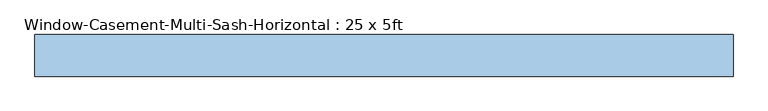
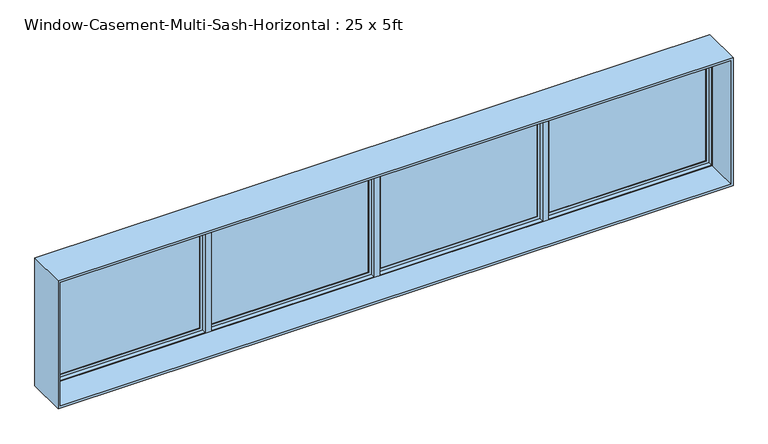
"""IFC4 building model written with IfcOpenShell, lengths in millimetres: window geometry, Window-Casement-Multi-Sash-Horizontal : 25 x 5ft."""

from ifc_helpers import new_model, si_unit, frame, origin, place, context, project, spatial, polyline, outline, extrude, faceted_brep, source, transform, mapped, element, save


def window_casement_multi_sash_horizontal_25_x_5ft_0e5d08e3(model_context):
    return source(origin(), model_context, "Body", "SolidModel", [
        extrude(outline(polyline([(2413.0, -1879.6), (939.8, -1879.6), (939.8, -25.4), (2413.0, -25.4), (2413.0, -1879.6)]), holes=[polyline([(2371.1296875, -67.2703125), (981.6703125, -67.2703125), (981.6703125, -1837.7296875), (2371.1296875, -1837.7296875), (2371.1296875, -67.2703125)])]), frame((0.0, 185.7375, 0.0), z_axis=(0.0, 1.0, 0.0), x_axis=(0.0, 0.0, 1.0)), (0.0, 0.0, 1.0), 31.75),
        extrude(outline(polyline([(2413.0, 25.4), (939.8, 25.4), (939.8, 1879.6), (2413.0, 1879.6), (2413.0, 25.4)]), holes=[polyline([(2371.1296875, 1837.7296875), (981.6703125, 1837.7296875), (981.6703125, 67.2703125), (2371.1296875, 67.2703125), (2371.1296875, 1837.7296875)])]), frame((0.0, 185.7375, 0.0), z_axis=(0.0, 1.0, 0.0), x_axis=(0.0, 0.0, 1.0)), (0.0, 0.0, 1.0), 31.75),
        faceted_brep([(-1930.4, 185.7375, 2413.0), (-3784.6, 185.7375, 2413.0), (-3784.6, 227.0125, 2413.0), (3784.6, 227.0125, 2413.0), (3784.6, 185.7375, 2413.0), (1930.4, 185.7375, 2413.0), (1930.4, 223.8375, 2413.0), (1879.6, 223.8375, 2413.0), (1879.6, 185.7375, 2413.0), (25.4, 185.7375, 2413.0), (25.4, 223.8375, 2413.0), (-25.4, 223.8375, 2413.0), (-25.4, 185.7375, 2413.0), (-1879.6, 185.7375, 2413.0), (-1879.6, 223.8375, 2413.0), (-1930.4, 223.8375, 2413.0), (-3774.4796875, 134.9375, 2402.8796875), (-3774.4796875, 185.7375, 2402.8796875), (-1940.5203125, 185.7375, 2402.8796875), (-1940.5203125, 134.9375, 2402.8796875), (3774.4796875, 185.7375, 2402.8796875), (3774.4796875, 134.9375, 2402.8796875), (1940.5203125, 134.9375, 2402.8796875), (1940.5203125, 185.7375, 2402.8796875), (-1869.4796875, 185.7375, 2402.8796875), (-35.5203125, 185.7375, 2402.8796875), (-35.5203125, 134.9375, 2402.8796875), (-1869.4796875, 134.9375, 2402.8796875), (35.5203125, 185.7375, 2402.8796875), (1869.4796875, 185.7375, 2402.8796875), (1869.4796875, 134.9375, 2402.8796875), (35.5203125, 134.9375, 2402.8796875), (-3784.6, -227.0125, 2413.0), (-3784.6, 134.9375, 2413.0), (3784.6, 134.9375, 2413.0), (3784.6, -227.0125, 2413.0), (-3810.0, 227.0125, 2438.4), (-3810.0, -227.0125, 2438.4), (3810.0, -227.0125, 2438.4), (3810.0, 227.0125, 2438.4), (3784.6, 227.0125, 939.8), (3784.6, 185.7375, 939.8), (3774.4796875, 185.7375, 949.9203125), (3774.4796875, 134.9375, 949.9203125), (3784.6, 134.9375, 939.8), (3784.6, -227.0125, 939.8), (3810.0, -227.0125, 914.4), (3810.0, 227.0125, 914.4), (1930.4, 185.7375, 939.8), (-3784.6, 227.0125, 939.8), (-3784.6, 185.7375, 939.8), (-1930.4, 185.7375, 939.8), (-1930.4, 223.8375, 939.8), (-1879.6, 223.8375, 939.8), (-1879.6, 185.7375, 939.8), (-25.4, 185.7375, 939.8), (-25.4, 223.8375, 939.8), (25.4, 223.8375, 939.8), (25.4, 185.7375, 939.8), (1879.6, 185.7375, 939.8), (1879.6, 223.8375, 939.8), (1930.4, 223.8375, 939.8), (1940.5203125, 185.7375, 949.9203125), (1940.5203125, 134.9375, 949.9203125), (-3774.4796875, 185.7375, 949.9203125), (-3774.4796875, 134.9375, 949.9203125), (-1940.5203125, 134.9375, 949.9203125), (-1940.5203125, 185.7375, 949.9203125), (-35.5203125, 185.7375, 949.9203125), (-1869.4796875, 185.7375, 949.9203125), (-1869.4796875, 134.9375, 949.9203125), (-35.5203125, 134.9375, 949.9203125), (1869.4796875, 185.7375, 949.9203125), (35.5203125, 185.7375, 949.9203125), (35.5203125, 134.9375, 949.9203125), (1869.4796875, 134.9375, 949.9203125), (-3784.6, 134.9375, 939.8), (-3784.6, -227.0125, 939.8), (-3810.0, -227.0125, 914.4), (-3810.0, 227.0125, 914.4)], [[[0, 1, 2, 3, 4, 5, 6, 7, 8, 9, 10, 11, 12, 13, 14, 15]], [[16, 17, 18, 19]], [[20, 21, 22, 23]], [[24, 25, 26, 27]], [[28, 29, 30, 31]], [[32, 33, 34, 35]], [[36, 37, 38, 39]], [[4, 3, 40, 41]], [[21, 20, 42, 43]], [[35, 34, 44, 45]], [[39, 38, 46, 47]], [[48, 41, 40, 49, 50, 51, 52, 53, 54, 55, 56, 57, 58, 59, 60, 61]], [[43, 42, 62, 63]], [[64, 65, 66, 67]], [[68, 69, 70, 71]], [[72, 73, 74, 75]], [[45, 44, 76, 77]], [[47, 46, 78, 79]], [[2, 1, 50, 49]], [[4, 41, 48, 5], [20, 23, 62, 42]], [[50, 1, 0, 51], [64, 67, 18, 17]], [[12, 55, 54, 13], [69, 68, 25, 24]], [[8, 59, 58, 9], [73, 72, 29, 28]], [[17, 16, 65, 64]], [[44, 34, 33, 76], [16, 19, 66, 65], [27, 26, 71, 70], [31, 30, 75, 74], [21, 43, 63, 22]], [[33, 32, 77, 76]], [[38, 37, 78, 46], [32, 35, 45, 77]], [[37, 36, 79, 78]], [[36, 39, 47, 79], [3, 2, 49, 40]], [[18, 67, 66, 19]], [[69, 24, 27, 70]], [[53, 14, 13, 54]], [[14, 53, 52, 15]], [[15, 52, 51, 0]], [[25, 68, 71, 26]], [[73, 28, 31, 74]], [[57, 10, 9, 58]], [[10, 57, 56, 11]], [[11, 56, 55, 12]], [[6, 61, 60, 7]], [[7, 60, 59, 8]], [[29, 72, 75, 30]], [[62, 23, 22, 63]], [[61, 6, 5, 48]]]),
        extrude(outline(polyline([(-67.2703125, 211.1375), (-67.2703125, 204.7875), (-1837.7296875, 204.7875), (-1837.7296875, 211.1375), (-67.2703125, 211.1375)])), frame((0.0, 0.0, 981.6703125), z_axis=(0.0, 0.0, 1.0), x_axis=(1.0, 0.0, 0.0)), (0.0, 0.0, 1.0), 1389.459375),
        extrude(outline(polyline([(-67.2703125, 198.4375), (-67.2703125, 192.0875), (-1837.7296875, 192.0875), (-1837.7296875, 198.4375), (-67.2703125, 198.4375)])), frame((0.0, 0.0, 981.6703125), z_axis=(0.0, 0.0, 1.0), x_axis=(1.0, 0.0, 0.0)), (0.0, 0.0, 1.0), 1389.459375),
        extrude(outline(polyline([(1837.7296875, 211.1375), (1837.7296875, 204.7875), (67.2703125, 204.7875), (67.2703125, 211.1375), (1837.7296875, 211.1375)])), frame((0.0, 0.0, 981.6703125), z_axis=(0.0, 0.0, 1.0), x_axis=(1.0, 0.0, 0.0)), (0.0, 0.0, 1.0), 1389.459375),
        extrude(outline(polyline([(1837.7296875, 198.4375), (1837.7296875, 192.0875), (67.2703125, 192.0875), (67.2703125, 198.4375), (1837.7296875, 198.4375)])), frame((0.0, 0.0, 981.6703125), z_axis=(0.0, 0.0, 1.0), x_axis=(1.0, 0.0, 0.0)), (0.0, 0.0, 1.0), 1389.459375),
        extrude(outline(polyline([(-1972.2703125, 211.1375), (-1972.2703125, 204.7875), (-3742.7296875, 204.7875), (-3742.7296875, 211.1375), (-1972.2703125, 211.1375)])), frame((0.0, 0.0, 981.6703125), z_axis=(0.0, 0.0, 1.0), x_axis=(1.0, 0.0, 0.0)), (0.0, 0.0, 1.0), 1389.459375),
        extrude(outline(polyline([(-1972.2703125, 198.4375), (-1972.2703125, 192.0875), (-3742.7296875, 192.0875), (-3742.7296875, 198.4375), (-1972.2703125, 198.4375)])), frame((0.0, 0.0, 981.6703125), z_axis=(0.0, 0.0, 1.0), x_axis=(1.0, 0.0, 0.0)), (0.0, 0.0, 1.0), 1389.459375),
        extrude(outline(polyline([(3742.7296875, 211.1375), (3742.7296875, 204.7875), (1972.2703125, 204.7875), (1972.2703125, 211.1375), (3742.7296875, 211.1375)])), frame((0.0, 0.0, 981.6703125), z_axis=(0.0, 0.0, 1.0), x_axis=(1.0, 0.0, 0.0)), (0.0, 0.0, 1.0), 1389.459375),
        extrude(outline(polyline([(3742.7296875, 198.4375), (3742.7296875, 192.0875), (1972.2703125, 192.0875), (1972.2703125, 198.4375), (3742.7296875, 198.4375)])), frame((0.0, 0.0, 981.6703125), z_axis=(0.0, 0.0, 1.0), x_axis=(1.0, 0.0, 0.0)), (0.0, 0.0, 1.0), 1389.459375),
        extrude(outline(polyline([(2413.0, -3784.6), (939.8, -3784.6), (939.8, -1930.4), (2413.0, -1930.4), (2413.0, -3784.6)]), holes=[polyline([(2371.1296875, -1972.2703125), (981.6703125, -1972.2703125), (981.6703125, -3742.7296875), (2371.1296875, -3742.7296875), (2371.1296875, -1972.2703125)])]), frame((0.0, 185.7375, 0.0), z_axis=(0.0, 1.0, 0.0), x_axis=(0.0, 0.0, 1.0)), (0.0, 0.0, 1.0), 31.75),
        extrude(outline(polyline([(2413.0, 1930.4), (939.8, 1930.4), (939.8, 3784.6), (2413.0, 3784.6), (2413.0, 1930.4)]), holes=[polyline([(2371.1296875, 3742.7296875), (981.6703125, 3742.7296875), (981.6703125, 1972.2703125), (2371.1296875, 1972.2703125), (2371.1296875, 3742.7296875)])]), frame((0.0, 185.7375, 0.0), z_axis=(0.0, 1.0, 0.0), x_axis=(0.0, 0.0, 1.0)), (0.0, 0.0, 1.0), 31.75),
    ])


if __name__ == "__main__":
    model = new_model("IFC4")
    model_context = context("Model", 3, world=origin())
    ifc_project = project(units=[si_unit("LENGTHUNIT", "METRE", prefix="MILLI")], contexts=[model_context])
    site = spatial("IfcSite", under=ifc_project)
    building = spatial("IfcBuilding", under=site)
    placement = place(None, origin())
    window_casement_multi_sash_horizontal_25_x_5ft_shape = window_casement_multi_sash_horizontal_25_x_5ft_0e5d08e3(model_context)
    element("IfcWindow", 1, ObjectType="Window-Casement-Multi-Sash-Horizontal : 25 x 5ft", at=placement, inside=building, context=model_context, shape_type="MappedRepresentation", body=[
        mapped(window_casement_multi_sash_horizontal_25_x_5ft_shape, transform((0.0, 0.0, 0.0), x_axis=(1.0, 0.0, 0.0), y_axis=(0.0, 1.0, 0.0), z_axis=(0.0, 0.0, 1.0))),
    ])
    save(model, "model.ifc")

# Revit data of these elements
# Type "Window-Casement-Multi-Sash-Horizontal : 25 x 5ft"
#   Type Mark = "WT-40"
#   Fire Rating = "0.5h"
#   Assembly Code = "B2020100"
#   Analytic Construction = "Double glazing - domestic"
#   Window Inset [instance default] = 0' - 0 5/8"
#   Wall Thickness [instance default] = 0' - 6"
#   Visual Light Transmittance = 0.81
#   Thermal Resistance (R) = 1.8146 (h·ft²·°F)/BTU
#   Solar Heat Gain Coefficient = 0.76
#   Rough Width = 25' - 0 1/2"
#   Rough Height = 5' - 0 1/2"
#   Open Window Width = 6' - 3"
#   Heat Transfer Coefficient (U) = 0.5511 BTU/(h·ft²·°F)
#   Height = 5' - 0"
#   Frame Gap 3 [instance default] = 0' - 1 83/128"
#   Frame Gap 2 [instance default] = 0' - 0 5/8"
#   Frame Gap 1 = 0' - 1 51/128"
#   Default Sill Height = 3' - 0"
#   Width = 25' - 0"
#   Define Thermal Properties by = 1
#   Frame Material = Metal - Aluminum
#   Glass Panel Material = Glass
#   Wall Closure = (empty or 0)
# Element 1 (IfcWindow, "Window-Casement-Multi-Sash-Horizontal : 25 x 5ft")
#   Wall Thickness = 1' - 5 7/8"
#   Materials on its faces: "Metal - Aluminum", "Glass"
# Materials
#   "Metal - Aluminum": class "Metal", colour RGB 247 247 247, transparency 0
#   "Glass": class "Glass", colour RGB 0 128 192, transparency 0.75, Description = "Soda Lime Glass", Cost = 0
